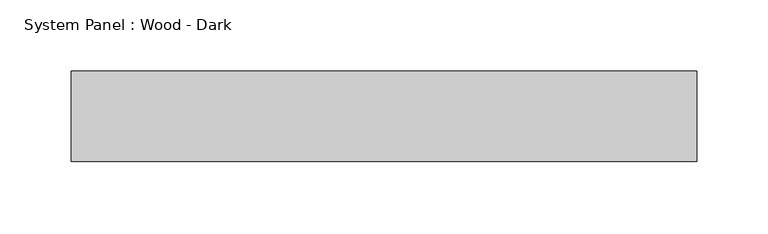
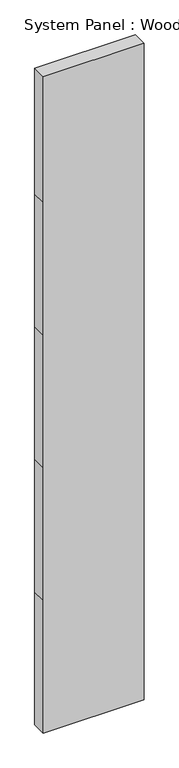
"""IFC4 building model written with IfcOpenShell, lengths in millimetres: plate geometry, System Panel : Wood - Dark."""

import ifcopenshell
import ifcopenshell.guid

model = None  # the IFC model being written
_history = None  # IfcOwnerHistory: only IFC2X3 demands one
_inside = {}  # id of a spatial element -> (the spatial element, [elements in it])
_under = {}  # id of a project, library or spatial element -> (it, [spatial elements below it])
_declared = {}  # id of a project -> (the project, [libraries it declares])
_typed = {}  # id of a type object -> (the type object, [elements of that type])
_made_of = {}  # id of a material, layer set ... -> (it, [elements and type objects made of it])


def new_model(schema):
    """Start an empty IFC model of exactly this schema.

    Asked for "IFC4X3", IfcOpenShell would pick the latest addendum, in which some entities
    have other attributes; the version numbers below select the first issue.
    IFC2X3 requires an IfcOwnerHistory on every rooted entity: one is made here for all.
    """
    global model, _history
    if schema == "IFC4X3":
        model = ifcopenshell.file(schema_version=(4, 3, 0, 0))
    else:
        model = ifcopenshell.file(schema=schema)
    _inside.clear()
    _under.clear()
    _declared.clear()
    _typed.clear()
    _made_of.clear()
    _history = None
    if model.schema == "IFC2X3":
        org = make("IfcOrganization", Name="unknown")
        user = make(
            "IfcPersonAndOrganization",
            ThePerson=make("IfcPerson", FamilyName="unknown"),
            TheOrganization=org,
        )
        app = make(
            "IfcApplication",
            ApplicationDeveloper=org,
            Version="unknown",
            ApplicationFullName="unknown",
            ApplicationIdentifier="unknown",
        )
        _history = make(
            "IfcOwnerHistory",
            OwningUser=user,
            OwningApplication=app,
            ChangeAction="ADDED",
            CreationDate=0,
        )
    return model


def make(cls, **values):
    """One entity of the class cls with the attributes given. An attribute that is None is left unset."""
    return model.create_entity(
        cls, **{name: value for name, value in values.items() if value is not None}
    )


def rooted(cls, **values):
    """An entity with a GlobalId (a new one), such as an element, a storey or a relation."""
    return make(cls, GlobalId=ifcopenshell.guid.new(), OwnerHistory=_history, **values)


def si_unit(unit_type, name, prefix=None):
    """IfcSIUnit, for example si_unit("LENGTHUNIT", "METRE", prefix="MILLI")."""
    return make("IfcSIUnit", UnitType=unit_type, Prefix=prefix, Name=name)


def assignment(units):
    """IfcUnitAssignment: the units of a project."""
    return None if units is None else make("IfcUnitAssignment", Units=units)


def point(xyz):
    """IfcCartesianPoint."""
    return None if xyz is None else make("IfcCartesianPoint", Coordinates=xyz)


def direction(xyz):
    """IfcDirection."""
    return None if xyz is None else make("IfcDirection", DirectionRatios=xyz)


def frame(location, z_axis=None, x_axis=None):
    """IfcAxis2Placement3D, a coordinate frame: its origin and axes. An axis left out is left unset."""
    return make(
        "IfcAxis2Placement3D",
        Location=point(location),
        Axis=direction(z_axis),
        RefDirection=direction(x_axis),
    )


def origin():
    """The frame at (0, 0, 0) with its axes left unset."""
    return frame((0.0, 0.0, 0.0))


def place(relative_to, where):
    """IfcLocalPlacement: puts the frame where relative to a parent placement (None: the world)."""
    return make(
        "IfcLocalPlacement", PlacementRelTo=relative_to, RelativePlacement=where
    )


def context(
    kind, dimensions, precision=None, world=None, true_north=None, identifier=None
):
    """IfcGeometricRepresentationContext, for example the 3D "Model" context."""
    return make(
        "IfcGeometricRepresentationContext",
        ContextIdentifier=identifier,
        ContextType=kind,
        CoordinateSpaceDimension=dimensions,
        Precision=precision,
        WorldCoordinateSystem=world,
        TrueNorth=true_north,
    )


def project(units=None, contexts=None):
    """IfcProject with its units and contexts."""
    return rooted(
        "IfcProject",
        Name="project",
        RepresentationContexts=contexts,
        UnitsInContext=assignment(units),
    )


def spatial(cls, under=None, at=None, **own):
    """A site, building, storey or space (cls), placed at a placement, below another one or the project."""
    s = rooted(cls, ObjectPlacement=at, **own)
    if under is not None:
        _under.setdefault(under.id(), (under, []))[1].append(s)
    return s


def polyline(points):
    """IfcPolyline through the points."""
    return make("IfcPolyline", Points=[point(p) for p in points])


def outline(outer, holes=None, kind="AREA"):
    """IfcArbitraryClosedProfileDef: a profile drawn as a closed curve; with holes, ...WithVoids."""
    if holes is None:
        return make("IfcArbitraryClosedProfileDef", ProfileType=kind, OuterCurve=outer)
    return make(
        "IfcArbitraryProfileDefWithVoids",
        ProfileType=kind,
        OuterCurve=outer,
        InnerCurves=holes,
    )


def extrude(swept, where, along, depth):
    """IfcExtrudedAreaSolid: the profile swept, set in the frame where, extruded along a direction by depth."""
    return make(
        "IfcExtrudedAreaSolid",
        SweptArea=swept,
        Position=where,
        ExtrudedDirection=direction(along),
        Depth=depth,
    )


def shape(context_of_items, identifier, shape_type, items):
    """IfcShapeRepresentation: the items that make up one representation, for example the "Body"."""
    return make(
        "IfcShapeRepresentation",
        ContextOfItems=context_of_items,
        RepresentationIdentifier=identifier,
        RepresentationType=shape_type,
        Items=items,
    )


def source(mapping_origin, context_of_items, identifier, shape_type, items):
    """IfcRepresentationMap: a shape defined once, which mapped items show again and again."""
    return make(
        "IfcRepresentationMap",
        MappingOrigin=mapping_origin,
        MappedRepresentation=shape(context_of_items, identifier, shape_type, items),
    )


def transform(
    local_origin,
    x_axis=None,
    y_axis=None,
    z_axis=None,
    scale=None,
    scale2=None,
    scale3=None,
    uniform=True,
):
    """IfcCartesianTransformationOperator3D, or its non-uniform kind. x_axis, y_axis, z_axis: its Axis1, 2, 3."""
    if uniform:
        return make(
            "IfcCartesianTransformationOperator3D",
            Axis1=direction(x_axis),
            Axis2=direction(y_axis),
            LocalOrigin=point(local_origin),
            Scale=scale,
            Axis3=direction(z_axis),
        )
    return make(
        "IfcCartesianTransformationOperator3DnonUniform",
        Axis1=direction(x_axis),
        Axis2=direction(y_axis),
        LocalOrigin=point(local_origin),
        Scale=scale,
        Axis3=direction(z_axis),
        Scale2=scale2,
        Scale3=scale3,
    )


def mapped(mapping_source, mapping_target):
    """IfcMappedItem: shows the shape of a source again, moved by a transform."""
    return make(
        "IfcMappedItem", MappingSource=mapping_source, MappingTarget=mapping_target
    )


def made_of(thing, what):
    """Note that an element or type object is made of a material, layer set ...; save() writes the relation."""
    if what is not None:
        _made_of.setdefault(what.id(), (what, []))[1].append(thing)
    return thing


def element(
    cls,
    number,
    at=None,
    inside=None,
    cuts=None,
    type_object=None,
    material=None,
    context=None,
    identifier="Body",
    shape_type=None,
    held_by="IfcProductDefinitionShape",
    body=None,
    shapes=None,
    **own,
):
    """One element of the class cls, such as IfcWall. Its Tag is "e" and its number.

    at: its placement. inside: the storey or other place that contains it. cuts: it is an
    opening in that element (IfcRelVoidsElement). A single representation is given by context,
    identifier, shape_type and body (its items); several are given by shapes. held_by: the class
    of the entity that holds the representations. save() writes the other relations.
    """
    e = rooted(cls, Tag="e%d" % number, ObjectPlacement=at, **own)
    if body is not None:
        shapes = [shape(context, identifier, shape_type, body)]
    if shapes is not None:
        e.Representation = make(held_by, Representations=shapes)
    if inside is not None:
        _inside.setdefault(inside.id(), (inside, []))[1].append(e)
    if cuts is not None:
        rooted(
            "IfcRelVoidsElement", RelatingBuildingElement=cuts, RelatedOpeningElement=e
        )
    if type_object is not None:
        _typed.setdefault(type_object.id(), (type_object, []))[1].append(e)
    return made_of(e, material)


def aggregate(whole, parts):
    """IfcRelAggregates: a whole, such as a stair, and the parts it consists of."""
    return rooted("IfcRelAggregates", RelatingObject=whole, RelatedObjects=parts)


def save(model, path):
    """Write the relations noted so far, then the file.

    IfcRelAggregates (storeys below a building ...), IfcRelContainedInSpatialStructure (elements
    in a storey), IfcRelDefinesByType, IfcRelAssociatesMaterial and IfcRelDeclares: one each for
    every whole, place, type object, material and project.
    """
    for whole, parts in _under.values():
        aggregate(whole, parts)
    for where, things in _inside.values():
        rooted(
            "IfcRelContainedInSpatialStructure",
            RelatedElements=things,
            RelatingStructure=where,
        )
    for kind, things in _typed.values():
        rooted("IfcRelDefinesByType", RelatedObjects=things, RelatingType=kind)
    for what, things in _made_of.values():
        rooted("IfcRelAssociatesMaterial", RelatedObjects=things, RelatingMaterial=what)
    for by, libraries in _declared.values():
        rooted("IfcRelDeclares", RelatingContext=by, RelatedDefinitions=libraries)
    model.write(path)


def system_panel_wood_dark_6d0ec728(model_context):
    return source(origin(), model_context, "Body", "SweptSolid", [
        extrude(outline(polyline([(0.0, -219.075), (0.0, 219.075), (609.6, 219.075), (1219.2, 219.075), (1828.8, 219.075), (2438.4, 219.075), (3016.25, 219.075), (3016.25, -219.075), (2438.4, -219.075), (1828.8, -219.075), (1219.2, -219.075), (609.6, -219.075), (0.0, -219.075)])), frame((0.0, -44.45, 0.0), z_axis=(0.0, 1.0, 0.0), x_axis=(0.0, 0.0, 1.0)), (0.0, 0.0, 1.0), 63.5),
    ])


if __name__ == "__main__":
    model = new_model("IFC4")
    model_context = context("Model", 3, world=origin())
    ifc_project = project(units=[si_unit("LENGTHUNIT", "METRE", prefix="MILLI")], contexts=[model_context])
    site = spatial("IfcSite", under=ifc_project)
    building = spatial("IfcBuilding", under=site)
    placement = place(None, origin())
    system_panel_wood_dark_shape = system_panel_wood_dark_6d0ec728(model_context)
    element("IfcPlate", 1, ObjectType="System Panel : Wood - Dark", at=placement, inside=building, context=model_context, shape_type="MappedRepresentation", body=[
        mapped(system_panel_wood_dark_shape, transform((0.0, 0.0, 0.0), x_axis=(1.0, 0.0, 0.0), y_axis=(0.0, 1.0, 0.0), z_axis=(0.0, 0.0, 1.0))),
    ])
    save(model, "model.ifc")

# Revit data of these elements
# Element 1 (IfcPlate, "System Panel : Wood - Dark")
#   Materials on its faces: "Wood Panel - Dark"
# Materials
#   "Wood Panel - Dark": class "Unassigned", colour RGB 57 19 6, transparency 0
